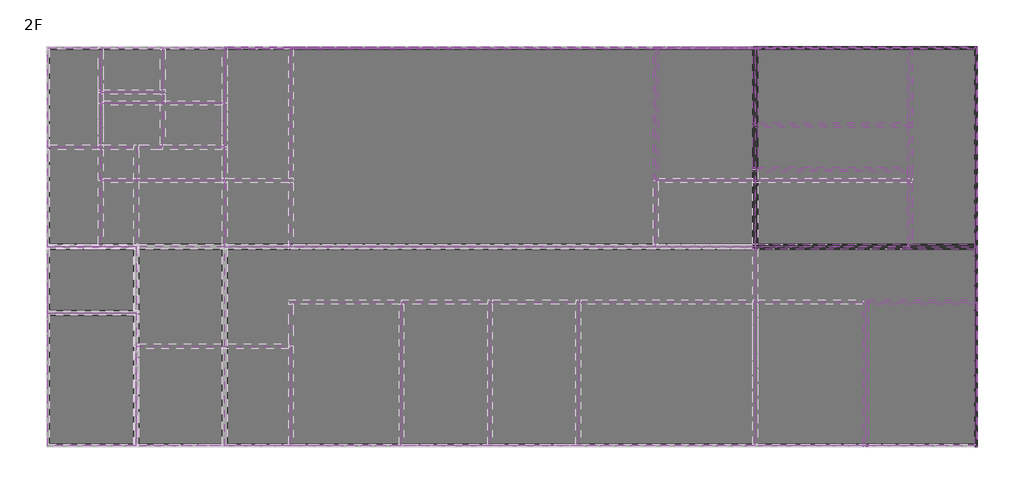
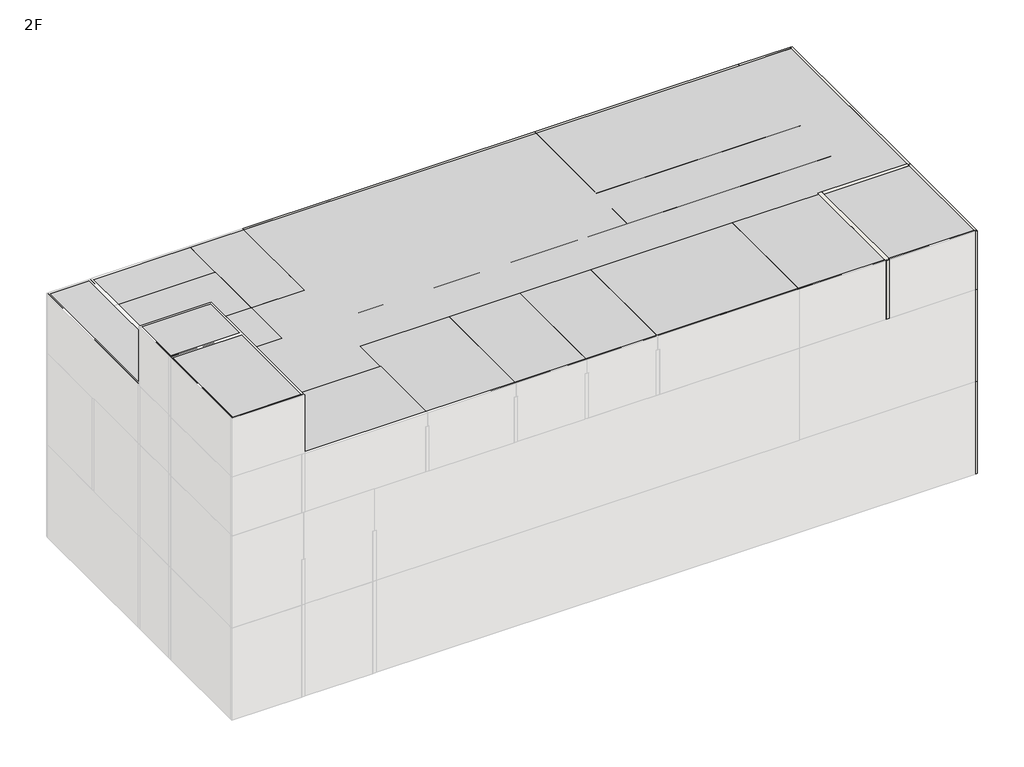
# One storey, part 3 of 3: 39 proxies, 28 walls.
# Revit data of these elements (continued)
# Type "Space Planning Box_hec : Space Planning Box_hec" (continued)
#   Assembly Code = "..."
#   ceiling height [instance default] = 0
#   Width [instance default] = 1524 mm
#   Program Area [instance default] = 0.00 m²
#   Length [instance default] = 1524 mm
#   Height [instance default] = 1524 mm
#   Area [instance default] = 2.32258 m²
#   Fill Color [instance default] = Cyan
#   Default Elevation = 0
# Type "WA211_Exterior-Cement Brick-90mm"
#   Type Comments = ""
#   Layers, outside or top first: 0 mm "A04AL081-00001_Skirt_Acrylic Emulsion Paint" (function 100); 0 mm "A04AL077-00001_Ext Wall Painting_Acrylic Emulsion Paint" (function 100); 12 mm "A04AS164-00001_Plastering_Ext" (function 4); 90 mm "A04AK073-00001_Concrete Brick_0.5B" (function 1); 12 mm "A04AS164-00002_Plastering_Int" (function 5); 0 mm "A04AL078-00002_Int Wall Painting_Water Emulsion Paint" (function 100); 0 mm "A04AL081-00001_Skirt_Acrylic Emulsion Paint" (function 100)
# Type "WA221_Interior-Cement Block-190mm"
#   Type Comments = ""
#   Layers, outside or top first: 0 mm "A04AL081-00001_Skirt_Acrylic Emulsion Paint" (function 100); 0 mm "A04AL078-00002_Int Wall Painting_Water Emulsion Paint" (function 100); 12 mm "A04AS164-00002_Plastering_Int" (function 2); 190 mm "A04AK069-00002_Reinforced Concrete Block_THK 100-200mm" (function 1); 12 mm "A04AS164-00002_Plastering_Int" (function 2); 0 mm "A04AL078-00002_Int Wall Painting_Water Emulsion Paint" (function 100); 0 mm "A04AL081-00001_Skirt_Acrylic Emulsion Paint" (function 100)
# Element 1 (IfcBuildingElementProxy, "Space Planning Box_hec : Space Planning Box_hec")
#   Room Name = "Staircase"
#   Interior Finish = "IW5..N/A..N/A,,N/A..N/A,,FL2..N/A,,CL1..N/A"
#   Exterior Finish = "N/A..N/A,,EW2..N/A..N/A"
#   Department = "PATHV1"
#   ceiling height = 0
#   Width = 4000 mm
#   Program Area = 24.00 m²
#   Length = 6000 mm
#   Height = 3500 mm
#   Area = 24.00 m²
#   Fill Color = Green
#   Phase Created = New Construction
#   Materials on its faces: "Green"
# Element 2 (IfcBuildingElementProxy, "Space Planning Box_hec : Space Planning Box_hec")
#   Room Name = "Staircase"
#   Interior Finish = "IW5..N/A..N/A,,WK3..N/A,,FL2..N/A,,CL1..N/A"
#   Exterior Finish = "RF1..N/A,,EW2..EW1..N/A"
#   Department = "PATHV1"
#   ceiling height = 0
#   Width = 4000 mm
#   Program Area = 0.00 m²
#   Length = 6000 mm
#   Height = 3500 mm
#   Area = 24.00 m²
#   Fill Color = Green
#   Phase Created = New Construction
#   Materials on its faces: "Green"
# Element 3 (IfcBuildingElementProxy, "Space Planning Box_hec : Space Planning Box_hec")
#   Room Name = "Electrical Room-1"
#   Interior Finish = "IW5..N/A..N/A,,WK1..N/A,,FL1..N/A,,CL1..N/A"
#   Exterior Finish = "N/A..N/A,,EW1..EW2..N/A"
#   Department = "CI"
#   ceiling height = 0
#   Width = 9000 mm
#   Program Area = 306.00 m²
#   Length = 32000 mm
#   Height = 5500 mm
#   Area = 288.00 m²
#   Fill Color = Yellow
#   Phase Created = New Construction
#   Materials on its faces: "Yellow"
# Element 4 (IfcBuildingElementProxy, "Space Planning Box_hec : Space Planning Box_hec")
#   Room Name = "Electrical Room-2"
#   Interior Finish = "IW5..N/A..N/A,,WK1..N/A,,FL1..N/A,,CL1..N/A"
#   Exterior Finish = "N/A..N/A,,EW1..EW2..N/A"
#   Department = "EL"
#   ceiling height = 0
#   Width = 9000 mm
#   Program Area = 288.00 m²
#   Length = 34000 mm
#   Height = 5500 mm
#   Area = 306.00 m²
#   Fill Color = Orange
#   Phase Created = New Construction
#   Materials on its faces: "Orange"
# Element 5 (IfcBuildingElementProxy, "Space Planning Box_hec : Space Planning Box_hec")
#   Room Name = "Electrical Room (GIS)"
#   Interior Finish = "IW5..N/A..N/A,,WK1..N/A,,FL1..N/A,,CL1..N/A"
#   Exterior Finish = "N/A..N/A,,EW1..EW2..N/A"
#   Department = "AR"
#   ceiling height = 0
#   Width = 9000 mm
#   Program Area = 90.00 m²
#   Length = 10000 mm
#   Height = 5500 mm
#   Area = 90.00 m²
#   Fill Color = Cyan
#   Phase Created = New Construction
#   Materials on its faces: "Cyan"
# Element 6 (IfcBuildingElementProxy, "Space Planning Box_hec : Space Planning Box_hec")
#   Room Name = "Lobby"
#   Interior Finish = "IW5..N/A..N/A,,WK3..N/A,,FL2..N/A,,CL3..N/A"
#   Exterior Finish = "N/A..N/A,,EW2..N/A..N/A"
#   Department = "AR"
#   ceiling height = 2700
#   Width = 4000 mm
#   Program Area = 36.00 m²
#   Length = 9000 mm
#   Height = 5500 mm
#   Area = 36.00 m²
#   Fill Color = Cyan
#   Phase Created = New Construction
#   Materials on its faces: "Cyan"
# Elements 7, 8 (IfcBuildingElementProxy, "Space Planning Box_hec : Space Planning Box_hec")
#   Room Name = "Elevator"
#   Interior Finish = "N/A..N/A..N/A,,N/A..N/A,,N/A..N/A,,N/A..N/A"
#   Exterior Finish = "N/A..N/A,,EW2..N/A..N/A"
#   Department = "PATHV2"
#   ceiling height = 0
#   Width = 4000 mm
#   Program Area = 12.00 m²
#   Length = 3000 mm
#   Height = 5500 mm
#   Area = 12.00 m²
#   Fill Color = Blue
#   Phase Created = New Construction
#   Materials on its faces: "Blue"
# Element 9 (IfcBuildingElementProxy, "Space Planning Box_hec : Space Planning Box_hec")
#   Room Name = "Staircase"
#   Interior Finish = "IW5..N/A..N/A,,WK3..N/A,,FL2..N/A,,CL1..N/A"
#   Exterior Finish = "N/A..N/A,,EW2..N/A..N/A"
#   Department = "PATHV1"
#   ceiling height = 0
#   Width = 4000 mm
#   Program Area = 24.00 m²
#   Length = 6000 mm
#   Height = 5500 mm
#   Area = 24.00 m²
#   Fill Color = Green
#   Phase Created = New Construction
#   Materials on its faces: "Green"
# Element 10 (IfcBuildingElementProxy, "Space Planning Box_hec : Space Planning Box_hec")
#   Room Name = "Staircase"
#   Interior Finish = "IW5..N/A..N/A,,WK3..N/A,,FL2..N/A,,CL1..N/A"
#   Exterior Finish = "N/A..N/A,,EW2..N/A..N/A"
#   Department = "PATHV1"
#   ceiling height = 2700
#   Width = 4000 mm
#   Program Area = 24.00 m²
#   Length = 6000 mm
#   Height = 5500 mm
#   Area = 24.00 m²
#   Fill Color = Green
#   Phase Created = New Construction
#   Materials on its faces: "Green"
# Element 11 (IfcBuildingElementProxy, "Space Planning Box_hec : Space Planning Box_hec")
#   Room Name = "Central Control Room"
#   Interior Finish = "IW5..N/A..N/A,,N/A..N/A,,FL5..N/A,,CL3..N/A"
#   Exterior Finish = "N/A..N/A,,EW1..N/A..N/A"
#   Department = "CI"
#   ceiling height = 3400
#   Width = 9000 mm
#   Program Area = 216.00 m²
#   Length = 24000 mm
#   Height = 5500 mm
#   Area = 216.00 m²
#   Fill Color = Yellow
#   Phase Created = New Construction
#   Materials on its faces: "Yellow"
# Element 12 (IfcBuildingElementProxy, "Space Planning Box_hec : Space Planning Box_hec")
#   Room Name = "Electronic Room"
#   Interior Finish = "IW5..N/A..N/A,,N/A..N/A,,FL5..N/A,,CL3..N/A"
#   Exterior Finish = "N/A..N/A,,EW1..N/A..N/A"
#   Department = "CI"
#   ceiling height = 3000
#   Width = 9000 mm
#   Program Area = 216.00 m²
#   Length = 24000 mm
#   Height = 5500 mm
#   Area = 216.00 m²
#   Fill Color = Yellow
#   Phase Created = New Construction
#   Materials on its faces: "Yellow"
# Element 13 (IfcBuildingElementProxy, "Space Planning Box_hec : Space Planning Box_hec")
#   Room Name = "Computer Room"
#   Interior Finish = "IW5..N/A..N/A,,N/A..N/A,,FL5..N/A,,CL3..N/A"
#   Exterior Finish = "N/A..N/A,,EW2..N/A..N/A"
#   Department = "AR"
#   ceiling height = 2700
#   Width = 7000 mm
#   Program Area = 24.50 m²
#   Length = 3500 mm
#   Height = 5500 mm
#   Area = 24.50 m²
#   Fill Color = Cyan
#   Phase Created = New Construction
#   Materials on its faces: "Cyan"
# Element 14 (IfcBuildingElementProxy, "Space Planning Box_hec : Space Planning Box_hec")
#   Room Name = "Electrical Room -3"
#   Interior Finish = "IW5..N/A..N/A,,N/A..N/A,,FL5,,CL3..N/A"
#   Exterior Finish = "N/A..N/A,,EW2..N/A..N/A"
#   Department = "EL"
#   ceiling height = 0
#   Width = 9000 mm
#   Program Area = 90.00 m²
#   Length = 10000 mm
#   Height = 5500 mm
#   Area = 90.00 m²
#   Fill Color = Orange
#   Phase Created = New Construction
#   Materials on its faces: "Orange"
# Element 15 (IfcBuildingElementProxy, "Space Planning Box_hec : Space Planning Box_hec")
#   Room Name = "Communication Room"
#   Interior Finish = "IW5..N/A..N/A,,N/A..N/A,,FL5..N/A,,CL3..N/A"
#   Exterior Finish = "N/A..N/A,,N/A..N/A..N/A"
#   Department = "CI"
#   ceiling height = 2700
#   Width = 7000 mm
#   Program Area = 24.50 m²
#   Length = 3500 mm
#   Height = 5500 mm
#   Area = 24.50 m²
#   Fill Color = Yellow
#   Phase Created = New Construction
#   Materials on its faces: "Yellow"
# Element 16 (IfcBuildingElementProxy, "Space Planning Box_hec : Space Planning Box_hec")
#   Room Name = "Duct Shaft"
#   Interior Finish = "N/A..N/A..N/A,,N/A..N/A,,N/A..N/A,,N/A..N/A"
#   Exterior Finish = "N/A..N/A,,EW2..N/A..N/A"
#   Department = "PATHV3"
#   ceiling height = 0
#   Width = 2400 mm
#   Program Area = 10.80 m²
#   Length = 4500 mm
#   Height = 5500 mm
#   Area = 10.80 m²
#   Fill Color = Lavender
#   Phase Created = New Construction
#   Materials on its faces: "Lavender"
# Element 17 (IfcBuildingElementProxy, "Space Planning Box_hec : Space Planning Box_hec")
#   Room Name = "Toilet (M)"
#   Interior Finish = "IW3..N/A..N/A,,N/A..N/A,,FL3..N/A,,CL4..N/A"
#   Exterior Finish = "N/A..N/A,,EW2..N/A..N/A"
#   Department = "AR"
#   ceiling height = 2700
#   Width = 4000 mm
#   Program Area = 18.00 m²
#   Length = 4500 mm
#   Height = 5500 mm
#   Area = 18.00 m²
#   Fill Color = Cyan
#   Phase Created = New Construction
#   Materials on its faces: "Cyan"
# Element 18 (IfcBuildingElementProxy, "Space Planning Box_hec : Space Planning Box_hec")
#   Room Name = "Toilet"
#   Interior Finish = "IW3..N/A..N/A,,N/A..N/A,,FL3..N/A,,CL4..N/A"
#   Exterior Finish = "N/A..N/A,,EW2..N/A..N/A"
#   Department = "AR"
#   ceiling height = 2700
#   Width = 2800 mm
#   Program Area = 12.60 m²
#   Length = 4500 mm
#   Height = 5500 mm
#   Area = 12.60 m²
#   Fill Color = Cyan
#   Phase Created = New Construction
#   Materials on its faces: "Cyan"
# Element 19 (IfcBuildingElementProxy, "Space Planning Box_hec : Space Planning Box_hec")
#   Room Name = "Shower"
#   Interior Finish = "IW3..N/A..N/A,,N/A..N/A,,FL3..N/A,,CL4..N/A"
#   Exterior Finish = "N/A..N/A,,EW2..N/A..N/A"
#   Department = "AR"
#   ceiling height = 2700
#   Width = 2800 mm
#   Program Area = 5.60 m²
#   Length = 2000 mm
#   Height = 5500 mm
#   Area = 5.60 m²
#   Fill Color = Cyan
#   Phase Created = New Construction
#   Materials on its faces: "Cyan"
# Element 20 (IfcBuildingElementProxy, "Space Planning Box_hec : Space Planning Box_hec")
#   Room Name = "Locker(F)"
#   Interior Finish = "IW5..N/A..N/A,,WK3..N/A,,FL2..N/A,,CL3..N/A"
#   Exterior Finish = "N/A..N/A,,N/A..N/A..N/A"
#   Department = "AR"
#   ceiling height = 2700
#   Width = 2800 mm
#   Program Area = 7.00 m²
#   Length = 2500 mm
#   Height = 5500 mm
#   Area = 7.00 m²
#   Fill Color = Cyan
#   Phase Created = New Construction
#   Materials on its faces: "Cyan"
# Element 21 (IfcBuildingElementProxy, "Space Planning Box_hec : Space Planning Box_hec")
#   Room Name = "Manager Office-1"
#   Interior Finish = "IW5..N/A..N/A,,WK3..N/A,,FL2..N/A,,CL3..N/A"
#   Exterior Finish = "RF1..N/A,,EW1..N/A..N/A"
#   Department = "AR"
#   ceiling height = 2700
#   Width = 6500 mm
#   Program Area = 26.00 m²
#   Length = 4000 mm
#   Height = 3500 mm
#   Area = 26.00 m²
#   Fill Color = Cyan
#   Phase Created = New Construction
#   Materials on its faces: "Cyan"
# Element 22 (IfcBuildingElementProxy, "Space Planning Box_hec : Space Planning Box_hec")
#   Room Name = "Manager Office-2"
#   Interior Finish = "IW5..N/A..N/A,,WK3..N/A,,FL2..N/A,,CL3..N/A"
#   Exterior Finish = "RF1..N/A,,EW1..N/A..N/A"
#   Department = "AR"
#   ceiling height = 2700
#   Width = 6500 mm
#   Program Area = 26.00 m²
#   Length = 4000 mm
#   Height = 3500 mm
#   Area = 26.00 m²
#   Fill Color = Cyan
#   Phase Created = New Construction
#   Materials on its faces: "Cyan"
# Element 23 (IfcBuildingElementProxy, "Space Planning Box_hec : Space Planning Box_hec")
#   Room Name = "Meeting Room-1"
#   Interior Finish = "IW5..N/A..N/A,,WK3..N/A,,FL2..N/A,,CL3..N/A"
#   Exterior Finish = "RF1..N/A,,EW1..EW2..N/A"
#   Department = "AR"
#   ceiling height = 2700
#   Width = 6000 mm
#   Program Area = 69.00 m²
#   Length = 11500 mm
#   Height = 3500 mm
#   Area = 69.00 m²
#   Fill Color = Cyan
#   Phase Created = New Construction
#   Materials on its faces: "Cyan"
# Element 24 (IfcBuildingElementProxy, "Space Planning Box_hec : Space Planning Box_hec")
#   Room Name = "Meeting Room-2"
#   Interior Finish = "IW5..N/A..N/A,,WK3..N/A,,FL2..N/A,,CL3..N/A"
#   Exterior Finish = "RF1..N/A,,EW1..N/A..N/A"
#   Department = "AR"
#   ceiling height = 2700
#   Width = 6500 mm
#   Program Area = 52.00 m²
#   Length = 8000 mm
#   Height = 3500 mm
#   Area = 52.00 m²
#   Fill Color = Cyan
#   Phase Created = New Construction
#   Materials on its faces: "Cyan"
# Element 25 (IfcBuildingElementProxy, "Space Planning Box_hec : Space Planning Box_hec")
#   Room Name = "Open Office"
#   Interior Finish = "IW5..N/A..N/A,,WK3..N/A,,FL2..N/A,,CL3..N/A"
#   Exterior Finish = "RF1..N/A,,EW1..N/A..N/A"
#   Department = "HV"
#   ceiling height = 2700
#   Width = 9000 mm
#   Program Area = 148.50 m²
#   Length = 16500 mm
#   Height = 3500 mm
#   Area = 148.50 m²
#   Fill Color = Lime
#   Phase Created = New Construction
#   Materials on its faces: "Lime"
# Element 26 (IfcBuildingElementProxy, "Space Planning Box_hec : Space Planning Box_hec")
#   Room Name = "Office-1"
#   Interior Finish = "IW5..N/A..N/A,,WK3..N/A,,FL2..N/A,,CL3..N/A"
#   Exterior Finish = "RF1..N/A,,EW2..N/A..N/A"
#   Department = "AR"
#   ceiling height = 2700
#   Width = 6500 mm
#   Program Area = 32.50 m²
#   Length = 5000 mm
#   Height = 3500 mm
#   Area = 32.50 m²
#   Fill Color = Cyan
#   Phase Created = New Construction
#   Materials on its faces: "Cyan"
# Element 27 (IfcBuildingElementProxy, "Space Planning Box_hec : Space Planning Box_hec")
#   Room Name = "Storage"
#   Interior Finish = "IW5..N/A..N/A,,WK3..N/A,,FL2..N/A,,CL3..N/A"
#   Exterior Finish = "RF1..N/A,,EW1..N/A..N/A"
#   Department = "AR"
#   ceiling height = 2700
#   Width = 6500 mm
#   Program Area = 32.50 m²
#   Length = 5000 mm
#   Height = 3500 mm
#   Area = 32.50 m²
#   Fill Color = Cyan
#   Phase Created = New Construction
#   Materials on its faces: "Cyan"
# Element 28 (IfcBuildingElementProxy, "Space Planning Box_hec : Space Planning Box_hec")
#   Room Name = "Fire Gas Room"
#   Interior Finish = "IW5..N/A..N/A,,WK1..N/A,,FL1..N/A,,N/A..N/A"
#   Exterior Finish = "RF1..N/A,,EW2..N/A..N/A"
#   Department = "FF"
#   ceiling height = 0
#   Width = 6500 mm
#   Program Area = 32.50 m²
#   Length = 5000 mm
#   Height = 3500 mm
#   Area = 32.50 m²
#   Fill Color = Red
#   Phase Created = New Construction
#   Materials on its faces: "Red"
# Element 29 (IfcBuildingElementProxy, "Space Planning Box_hec : Space Planning Box_hec")
#   Room Name = "Document Room"
#   Interior Finish = "IW5..N/A..N/A,,WK3..N/A,,FL2..N/A,,CL3..N/A"
#   Exterior Finish = "RF1..N/A,,N/A..N/A..N/A"
#   Department = "AR"
#   ceiling height = 2700
#   Width = 3000 mm
#   Program Area = 34.50 m²
#   Length = 11500 mm
#   Height = 3500 mm
#   Area = 34.50 m²
#   Fill Color = Cyan
#   Phase Created = New Construction
#   Materials on its faces: "Cyan"
# Element 30 (IfcBuildingElementProxy, "Space Planning Box_hec : Space Planning Box_hec")
#   Room Name = "Break Room"
#   Interior Finish = "IW5..N/A..N/A,,WK3..N/A,,FL2..N/A,,CL3..N/A"
#   Exterior Finish = "RF1..N/A,,EW2..N/A..N/A"
#   Department = "AR"
#   ceiling height = 2700
#   Width = 4500 mm
#   Program Area = 31.50 m²
#   Length = 7000 mm
#   Height = 3500 mm
#   Area = 31.50 m²
#   Fill Color = Cyan
#   Phase Created = New Construction
#   Materials on its faces: "Cyan"
# Element 31 (IfcBuildingElementProxy, "Space Planning Box_hec : Space Planning Box_hec")
#   Room Name = "Toilet"
#   Interior Finish = "IW3..N/A..N/A,,N/A..N/A,,FL3..N/A,,CL4..N/A"
#   Exterior Finish = "RF1..N/A,,N/A..N/A..N/A"
#   Department = "AR"
#   ceiling height = 2700
#   Width = 3500 mm
#   Program Area = 19.60 m²
#   Length = 5600 mm
#   Height = 3500 mm
#   Area = 19.60 m²
#   Fill Color = Cyan
#   Phase Created = New Construction
#   Materials on its faces: "Cyan"
# Element 32 (IfcBuildingElementProxy, "Space Planning Box_hec : Space Planning Box_hec")
#   Room Name = "Shower"
#   Interior Finish = "IW3..N/A..N/A,,N/A..N/A,,FL3..N/A,,CL4..N/A"
#   Exterior Finish = "RF1..N/A,,EW2..N/A..N/A"
#   Department = "AR"
#   ceiling height = 2700
#   Width = 2500 mm
#   Program Area = 14.00 m²
#   Length = 5600 mm
#   Height = 3500 mm
#   Area = 14.00 m²
#   Fill Color = Cyan
#   Phase Created = New Construction
#   Materials on its faces: "Cyan"
# Element 33 (IfcBuildingElementProxy, "Space Planning Box_hec : Space Planning Box_hec")
#   Room Name = "Locker(M)"
#   Interior Finish = "IW5..N/A..N/A,,WK3..N/A,,FL2..N/A,,CL3..N/A"
#   Exterior Finish = "RF1..N/A,,EW1..N/A..N/A"
#   Department = "AR"
#   ceiling height = 2700
#   Width = 6000 mm
#   Program Area = 18.00 m²
#   Length = 3000 mm
#   Height = 3500 mm
#   Area = 18.00 m²
#   Fill Color = Cyan
#   Phase Created = New Construction
#   Materials on its faces: "Cyan"
# Element 34 (IfcBuildingElementProxy, "Space Planning Box_hec : Space Planning Box_hec")
#   Room Name = "Toilet(F)"
#   Interior Finish = "IW3..N/A..N/A,,N/A..N/A,,FL3..N/A,,CL4..N/A"
#   Exterior Finish = "RF1..N/A,,N/A..N/A..N/A"
#   Department = "AR"
#   ceiling height = 2700
#   Width = 3000 mm
#   Program Area = 16.80 m²
#   Length = 5600 mm
#   Height = 3500 mm
#   Area = 16.80 m²
#   Fill Color = Cyan
#   Phase Created = New Construction
#   Materials on its faces: "Cyan"
# Element 35 (IfcBuildingElementProxy, "Space Planning Box_hec : Space Planning Box_hec")
#   Room Name = "Duct Shaft"
#   Interior Finish = "N/A..N/A..N/A,,N/A..N/A,,N/A..N/A,,N/A..N/A"
#   Exterior Finish = "RF1..N/A,,EW2..N/A..N/A"
#   Department = "PATHV3"
#   ceiling height = 0
#   Width = 2400 mm
#   Program Area = 21.60 m²
#   Length = 9000 mm
#   Height = 3500 mm
#   Area = 21.60 m²
#   Fill Color = Lavender
#   Phase Created = New Construction
#   Materials on its faces: "Lavender"
# Element 36 (IfcBuildingElementProxy, "Space Planning Box_hec : Space Planning Box_hec")
#   Room Name = "Elevator"
#   Interior Finish = "N/A..N/A..N/A,,N/A..N/A,,N/A..N/A,,N/A..N/A"
#   Exterior Finish = "N/A..N/A,,EW2..N/A..N/A"
#   Department = "PATHV2"
#   ceiling height = 0
#   Width = 4000 mm
#   Program Area = 12.00 m²
#   Length = 3000 mm
#   Height = 3500 mm
#   Area = 12.00 m²
#   Fill Color = Blue
#   Phase Created = New Construction
#   Materials on its faces: "Blue"
# Element 37 (IfcBuildingElementProxy, "Space Planning Box_hec : Space Planning Box_hec")
#   Room Name = "Elevator"
#   Interior Finish = "N/A..N/A..N/A,,N/A..N/A,,N/A..N/A,,N/A..N/A"
#   Exterior Finish = "RF1..N/A,,EW2..EW1..N/A"
#   Department = "PATHV2"
#   ceiling height = 0
#   Width = 4000 mm
#   Program Area = 0.00 m²
#   Length = 3000 mm
#   Height = 3500 mm
#   Area = 12.00 m²
#   Fill Color = Blue
#   Phase Created = New Construction
#   Materials on its faces: "Blue"
# Element 38 (IfcBuildingElementProxy, "Space Planning Box_hec : Space Planning Box_hec")
#   Room Name = "Corridor"
#   Interior Finish = "IW5..N/A..N/A,,WK3..N/A,,FL2..N/A,,CL3..N/A"
#   Exterior Finish = "N/A..N/A,,EW2..N/A..N/A"
#   Department = "AR"
#   ceiling height = 2700
#   Width = 42000 mm
#   Program Area = 54.00 m²
#   Length = 18000 mm
#   Height = 5500 mm
#   Area = 756.00 m²
#   Fill Color = Cyan
#   Phase Created = New Construction
#   Materials on its faces: "Cyan"
# Element 39 (IfcBuildingElementProxy, "Space Planning Box_hec : Space Planning Box_hec")
#   Room Name = "Corridor"
#   Interior Finish = "IW5..N/A..N/A,,WK3..N/A,,FL2..N/A,,CL3..N/A"
#   Exterior Finish = "RF1..N/A,,EW2..N/A..N/A"
#   Department = "AR"
#   ceiling height = 2700
#   Width = 18000 mm
#   Program Area = 95.00 m²
#   Length = 42000 mm
#   Height = 3500 mm
#   Area = 756.00 m²
#   Fill Color = Cyan
#   Phase Created = New Construction
#   Materials on its faces: "Cyan"
# Elements 40, 41 (IfcWall, "WA211_Exterior-Cement Brick-90mm")
#   Top Offset = 0 mm
#   Base Offset = 0 mm
#   Unconnected Height = 5500 mm
#   wall height = 5500 mm
#   Phase Created = New Construction
#   Base Constraint = 2F
#   Materials on its faces: "Default Wall", "A04AS164-00001_Plastering_Ext", "A04AS164-00002_Plastering_Int"
# Element 42 (IfcWall, "WA211_Exterior-Cement Brick-90mm")
#   Top Offset = 0 mm
#   Base Offset = 0 mm
#   Unconnected Height = 5500 mm
#   wall height = 5500 mm
#   Phase Created = New Construction
#   Base Constraint = 2F
#   Materials on its faces: "Default Wall", "A04AS164-00002_Plastering_Int", "A04AS164-00001_Plastering_Ext"
# Elements 43, 44, 47 (IfcWall, "WA211_Exterior-Cement Brick-90mm")
#   Top Offset = 0 mm
#   Base Offset = 0 mm
#   Unconnected Height = 5500 mm
#   wall height = 5500 mm
#   Phase Created = New Construction
#   Base Constraint = 3F
#   Materials on its faces: "Default Wall", "A04AS164-00002_Plastering_Int", "A04AS164-00001_Plastering_Ext"
# Elements 45, 46 (IfcWall, "WA211_Exterior-Cement Brick-90mm")
#   Top Offset = 0 mm
#   Base Offset = 0 mm
#   Unconnected Height = 5500 mm
#   wall height = 5500 mm
#   Phase Created = New Construction
#   Base Constraint = 3F
#   Materials on its faces: "Default Wall", "A04AS164-00001_Plastering_Ext", "A04AS164-00002_Plastering_Int"
# Elements 48, 49, 52 (IfcWall, "WA211_Exterior-Cement Brick-90mm")
#   Top Offset = 0 mm
#   Base Offset = 0 mm
#   Unconnected Height = 3500 mm
#   wall height = 3500 mm
#   Phase Created = New Construction
#   Base Constraint = 4F
#   Materials on its faces: "Default Wall", "A04AS164-00002_Plastering_Int", "A04AS164-00001_Plastering_Ext"
# Elements 50, 51 (IfcWall, "WA211_Exterior-Cement Brick-90mm")
#   Top Offset = 0 mm
#   Base Offset = 0 mm
#   Unconnected Height = 3500 mm
#   wall height = 3500 mm
#   Phase Created = New Construction
#   Base Constraint = 4F
#   Materials on its faces: "Default Wall", "A04AS164-00001_Plastering_Ext", "A04AS164-00002_Plastering_Int"
# Element 53 (IfcWall, "WA221_Interior-Cement Block-190mm")
#   Top Offset = 0 mm
#   Base Offset = 0 mm
#   Unconnected Height = 5500 mm
#   wall height = 5500 mm
#   Phase Created = New Construction
#   Base Constraint = 2F
#   Materials on its faces: "A04AS164-00002_Plastering_Int", "Default Wall", "A04AS164-00001_Plastering_Ext"
# Element 54 (IfcWall, "WA221_Interior-Cement Block-190mm")
#   Top Offset = 0 mm
#   Base Offset = 0 mm
#   Unconnected Height = 5500 mm
#   wall height = 5500 mm
#   Phase Created = New Construction
#   Base Constraint = 2F
#   Materials on its faces: "Default Wall", "A04AS164-00002_Plastering_Int"
# Element 55 (IfcWall, "WA221_Interior-Cement Block-190mm")
#   Top Offset = 0 mm
#   Base Offset = 0 mm
#   Unconnected Height = 3400 mm
#   wall height = 3400 mm
#   Phase Created = New Construction
#   Base Constraint = 3F
#   Materials on its faces: "Default Wall", "A04AS164-00002_Plastering_Int", "A04AS164-00001_Plastering_Ext"
# Element 56 (IfcWall, "WA221_Interior-Cement Block-190mm")
#   Top Offset = 0 mm
#   Base Offset = 0 mm
#   Unconnected Height = 3400 mm
#   wall height = 3400 mm
#   Phase Created = New Construction
#   Base Constraint = 3F
#   Materials on its faces: "Default Wall", "A04AS164-00002_Plastering_Int"
# Elements 57, 61, 62 (IfcWall, "WA221_Interior-Cement Block-190mm")
#   Top Offset = 0 mm
#   Base Offset = 0 mm
#   Unconnected Height = 2700 mm
#   wall height = 2700 mm
#   Phase Created = New Construction
#   Base Constraint = 3F
#   Materials on its faces: "A04AS164-00002_Plastering_Int", "Default Wall"
# Element 58 (IfcWall, "WA221_Interior-Cement Block-190mm")
#   Top Offset = 0 mm
#   Base Offset = 0 mm
#   Unconnected Height = 2700 mm
#   wall height = 2700 mm
#   Phase Created = New Construction
#   Base Constraint = 3F
#   Materials on its faces: "Default Wall", "A04AS164-00002_Plastering_Int", "A04AS164-00001_Plastering_Ext"
# Elements 59, 60 (IfcWall, "WA221_Interior-Cement Block-190mm")
#   Top Offset = 0 mm
#   Base Offset = 0 mm
#   Unconnected Height = 5500 mm
#   wall height = 5500 mm
#   Phase Created = New Construction
#   Base Constraint = 3F
#   Materials on its faces: "Default Wall", "A04AS164-00002_Plastering_Int"
# Elements 63, 64 (IfcWall, "WA221_Interior-Cement Block-190mm")
#   Top Offset = 0 mm
#   Base Offset = 0 mm
#   Unconnected Height = 2700 mm
#   wall height = 2700 mm
#   Phase Created = New Construction
#   Base Constraint = 4F
#   Materials on its faces: "Default Wall", "A04AS164-00002_Plastering_Int", "A04AS164-00001_Plastering_Ext"
# Element 65 (IfcWall, "WA221_Interior-Cement Block-190mm")
#   Top Offset = 0 mm
#   Base Offset = 0 mm
#   Unconnected Height = 3500 mm
#   wall height = 3500 mm
#   Phase Created = New Construction
#   Base Constraint = 4F
#   Materials on its faces: "A04AS164-00002_Plastering_Int", "Default Wall", "A04AS164-00001_Plastering_Ext"
# Element 66 (IfcWall, "WA221_Interior-Cement Block-190mm")
#   Top Offset = 0 mm
#   Base Offset = 0 mm
#   Unconnected Height = 3500 mm
#   wall height = 3500 mm
#   Phase Created = New Construction
#   Base Constraint = 4F
#   Materials on its faces: "Default Wall", "A04AS164-00002_Plastering_Int"
# Element 67 (IfcWall, "WA221_Interior-Cement Block-190mm")
#   Top Offset = 0 mm
#   Base Offset = 0 mm
#   Unconnected Height = 2700 mm
#   wall height = 2700 mm
#   Phase Created = New Construction
#   Base Constraint = 4F
#   Materials on its faces: "A04AS164-00002_Plastering_Int", "Default Wall"
# Materials
#   "Cyan": class "Generic", colour RGB 0 255 255, transparency 0.2, Cost = 0
#   "A04AL081-00001_Skirt_Acrylic Emulsion Paint": class "Finish", colour RGB 128 128 64, transparency 0, Description = "Plastic", W00) Work Master Code = "A04AL081-00001", W01) Work Master_Lv1 = "Finishing Work", W02) Work Master_Lv2 = "Painting Work", W03) Work Master_Spec.1 = "Skirt Painting", W04) Work Master_Spec.2 = "Acrylic Emulsion Paint", W05) Work Master_Spec.3 = "100mm≤H<150mm", Cost = 0
#   "A04AL077-00001_Ext Wall Painting_Acrylic Emulsion Paint": class "Finish", colour RGB 128 128 64, transparency 0, Description = "Plastic", W00) Work Master Code = "A04AL077-00001", W01) Work Master_Lv1 = "Finishing Work", W02) Work Master_Lv2 = "Painting Work", W03) Work Master_Spec.1 = "External Wall Painting", W04) Work Master_Spec.2 = "Acrylic Emulsion Paint", Cost = 0
#   "A04AS164-00001_Plastering_Ext": class "Concrete", colour RGB 183 186 184, transparency 0, W00) Work Master Code = "A04AS164-00001", W01) Work Master_Lv1 = "Finishing Work", W02) Work Master_Lv2 = "Plastering Work", W03) Work Master_Spec.1 = "Plastering", W04) Work Master_Spec.2 = "for External Masonry Wall", Cost = 0
#   "A04AK073-00001_Concrete Brick_0.5B": class "Concrete", colour RGB 180 180 180, transparency 0, Description = "Conc. Block", W00) Work Master Code = "A04AK073-00001", W01) Work Master_Lv1 = "Finishing Work", W02) Work Master_Lv2 = "Masonry Work", W03) Work Master_Spec.1 = "Concrete Brick", W04) Work Master_Spec.2 = "[0.5B] w/ All Reinf.(Lath, Steel Tie, Anchor Bar, Mortar, ETC.), Filler, Sealant, Lintel/Sill for Opening, ETC.", Cost = 0
#   "A04AS164-00002_Plastering_Int": class "Concrete", colour RGB 183 186 184, transparency 0, Description = "LATEX PAINT ON THK.15 CEMENT PLASTER", W00) Work Master Code = "A04AS164-00002", W01) Work Master_Lv1 = "Finishing Work", W02) Work Master_Lv2 = "Plastering Work", W03) Work Master_Spec.1 = "Plastering", W04) Work Master_Spec.2 = "for Internal Masonry Wall", Cost = 0
#   "A04AL078-00002_Int Wall Painting_Water Emulsion Paint": class "Finish", colour RGB 128 128 64, transparency 0, Description = "Plastic", W00) Work Master Code = "A04AL078-00002", W01) Work Master_Lv1 = "Finishing Work", W02) Work Master_Lv2 = "Painting Work", W03) Work Master_Spec.1 = "Internal Wall Painting", W04) Work Master_Spec.2 = "Water Emulsion Paint", Cost = 0
#   "A04AK069-00002_Reinforced Concrete Block_THK 100-200mm": class "Concrete", colour RGB 180 180 180, transparency 0, Description = "Conc. Block", W00) Work Master Code = "A04AK069-00002", W01) Work Master_Lv1 = "Finishing Work", W02) Work Master_Lv2 = "Masonry Work", W03) Work Master_Spec.1 = "Reinforced Concrete Block", W04) Work Master_Spec.2 = "w/ All Reinf.(Lath, Steel Tie, Anchor Bar, Mortar, ETC.), Filler, Sealant, Lintel/Sill for Opening, ETC.", W05) Work Master_Spec.3 = "100mm<THK≤200mm", Cost = 0
#   "Green": class "Generic", colour RGB 0 128 0, transparency 0.2, Cost = 0
#   "Yellow": class "Generic", colour RGB 255 255 0, transparency 0.2, Cost = 0
#   "Orange": class "Generic", colour RGB 255 165 0, transparency 0.2, Cost = 0
#   "Blue": class "Generic", colour RGB 0 0 255, transparency 0.2, Cost = 0
#   "Lavender": class "Generic", colour RGB 186 85 211, transparency 0.2, Cost = 0
#   "Lime": class "Generic", colour RGB 0 255 0, transparency 0.2, Cost = 0
#   "Red": class "Generic", colour RGB 255 0 0, transparency 0.2, Cost = 0
#   "Default Wall": class "Miscellaneous", colour RGB 80 80 80, transparency 0
